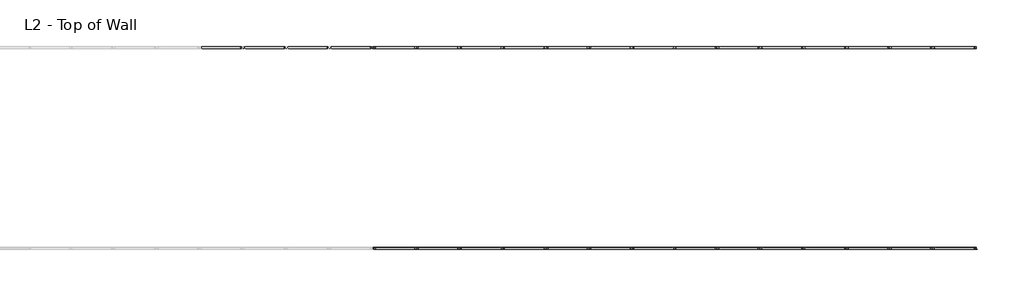
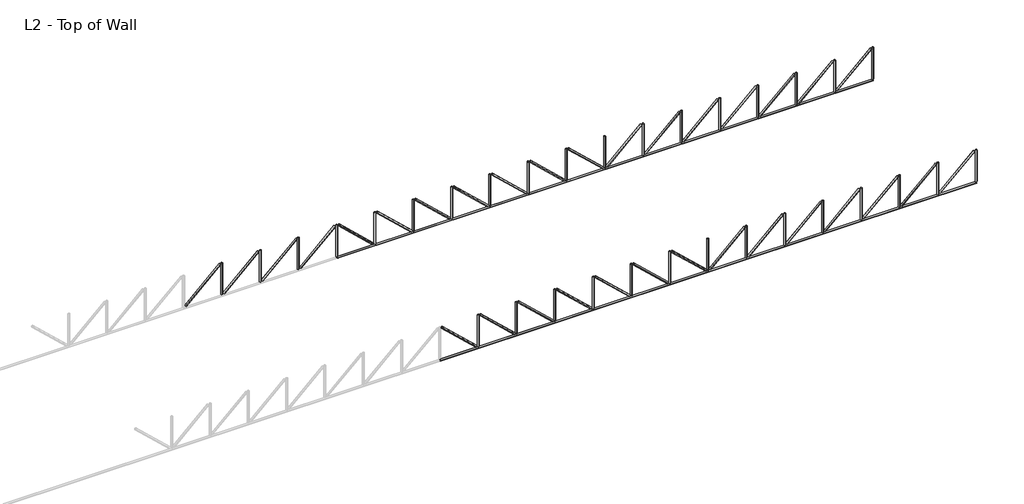
# One storey, part 4 of 4: 98 beams.
"""IFC4 building model written with IfcOpenShell, lengths in millimetres."""

import ifcopenshell
import ifcopenshell.guid

model = None  # the IFC model being written
_history = None  # IfcOwnerHistory: only IFC2X3 demands one
_inside = {}  # id of a spatial element -> (the spatial element, [elements in it])
_under = {}  # id of a project, library or spatial element -> (it, [spatial elements below it])
_declared = {}  # id of a project -> (the project, [libraries it declares])
_typed = {}  # id of a type object -> (the type object, [elements of that type])
_made_of = {}  # id of a material, layer set ... -> (it, [elements and type objects made of it])


def new_model(schema):
    """Start an empty IFC model of exactly this schema.

    Asked for "IFC4X3", IfcOpenShell would pick the latest addendum, in which some entities
    have other attributes; the version numbers below select the first issue.
    IFC2X3 requires an IfcOwnerHistory on every rooted entity: one is made here for all.
    """
    global model, _history
    if schema == "IFC4X3":
        model = ifcopenshell.file(schema_version=(4, 3, 0, 0))
    else:
        model = ifcopenshell.file(schema=schema)
    _inside.clear()
    _under.clear()
    _declared.clear()
    _typed.clear()
    _made_of.clear()
    _history = None
    if model.schema == "IFC2X3":
        org = make("IfcOrganization", Name="unknown")
        user = make(
            "IfcPersonAndOrganization",
            ThePerson=make("IfcPerson", FamilyName="unknown"),
            TheOrganization=org,
        )
        app = make(
            "IfcApplication",
            ApplicationDeveloper=org,
            Version="unknown",
            ApplicationFullName="unknown",
            ApplicationIdentifier="unknown",
        )
        _history = make(
            "IfcOwnerHistory",
            OwningUser=user,
            OwningApplication=app,
            ChangeAction="ADDED",
            CreationDate=0,
        )
    return model


def make(cls, **values):
    """One entity of the class cls with the attributes given. An attribute that is None is left unset."""
    return model.create_entity(
        cls, **{name: value for name, value in values.items() if value is not None}
    )


def rooted(cls, **values):
    """An entity with a GlobalId (a new one), such as an element, a storey or a relation."""
    return make(cls, GlobalId=ifcopenshell.guid.new(), OwnerHistory=_history, **values)


def si_unit(unit_type, name, prefix=None):
    """IfcSIUnit, for example si_unit("LENGTHUNIT", "METRE", prefix="MILLI")."""
    return make("IfcSIUnit", UnitType=unit_type, Prefix=prefix, Name=name)


def assignment(units):
    """IfcUnitAssignment: the units of a project."""
    return None if units is None else make("IfcUnitAssignment", Units=units)


def point(xyz):
    """IfcCartesianPoint."""
    return None if xyz is None else make("IfcCartesianPoint", Coordinates=xyz)


def direction(xyz):
    """IfcDirection."""
    return None if xyz is None else make("IfcDirection", DirectionRatios=xyz)


def frame(location, z_axis=None, x_axis=None):
    """IfcAxis2Placement3D, a coordinate frame: its origin and axes. An axis left out is left unset."""
    return make(
        "IfcAxis2Placement3D",
        Location=point(location),
        Axis=direction(z_axis),
        RefDirection=direction(x_axis),
    )


def frame_2d(location, x_axis=None):
    """IfcAxis2Placement2D, a coordinate frame in the plane: its origin and x axis."""
    return make(
        "IfcAxis2Placement2D", Location=point(location), RefDirection=direction(x_axis)
    )


def origin():
    """The frame at (0, 0, 0) with its axes left unset."""
    return frame((0.0, 0.0, 0.0))


def origin_2d():
    """The frame at (0, 0) in the plane with its x axis left unset."""
    return frame_2d((0.0, 0.0))


def place(relative_to, where):
    """IfcLocalPlacement: puts the frame where relative to a parent placement (None: the world)."""
    return make(
        "IfcLocalPlacement", PlacementRelTo=relative_to, RelativePlacement=where
    )


def context(
    kind, dimensions, precision=None, world=None, true_north=None, identifier=None
):
    """IfcGeometricRepresentationContext, for example the 3D "Model" context."""
    return make(
        "IfcGeometricRepresentationContext",
        ContextIdentifier=identifier,
        ContextType=kind,
        CoordinateSpaceDimension=dimensions,
        Precision=precision,
        WorldCoordinateSystem=world,
        TrueNorth=true_north,
    )


def project(units=None, contexts=None):
    """IfcProject with its units and contexts."""
    return rooted(
        "IfcProject",
        Name="project",
        RepresentationContexts=contexts,
        UnitsInContext=assignment(units),
    )


def spatial(cls, under=None, at=None, **own):
    """A site, building, storey or space (cls), placed at a placement, below another one or the project."""
    s = rooted(cls, ObjectPlacement=at, **own)
    if under is not None:
        _under.setdefault(under.id(), (under, []))[1].append(s)
    return s


def circle_curve(where, radius):
    """IfcCircle in the frame where."""
    return make("IfcCircle", Position=where, Radius=radius)


def trimmed(basis, trim1, trim2, sense, master):
    """IfcTrimmedCurve: the piece of a basis curve between two trims."""
    return make(
        "IfcTrimmedCurve",
        BasisCurve=basis,
        Trim1=trim1,
        Trim2=trim2,
        SenseAgreement=sense,
        MasterRepresentation=master,
    )


def segment(curve, same_sense, transition):
    """IfcCompositeCurveSegment."""
    return make(
        "IfcCompositeCurveSegment",
        Transition=transition,
        SameSense=same_sense,
        ParentCurve=curve,
    )


def composite_curve(segments, self_intersect=None):
    """IfcCompositeCurve: segments joined end to end."""
    return make("IfcCompositeCurve", Segments=segments, SelfIntersect=self_intersect)


def outline(outer, holes=None, kind="AREA"):
    """IfcArbitraryClosedProfileDef: a profile drawn as a closed curve; with holes, ...WithVoids."""
    if holes is None:
        return make("IfcArbitraryClosedProfileDef", ProfileType=kind, OuterCurve=outer)
    return make(
        "IfcArbitraryProfileDefWithVoids",
        ProfileType=kind,
        OuterCurve=outer,
        InnerCurves=holes,
    )


def extrude(swept, where, along, depth):
    """IfcExtrudedAreaSolid: the profile swept, set in the frame where, extruded along a direction by depth."""
    return make(
        "IfcExtrudedAreaSolid",
        SweptArea=swept,
        Position=where,
        ExtrudedDirection=direction(along),
        Depth=depth,
    )


def shape(context_of_items, identifier, shape_type, items):
    """IfcShapeRepresentation: the items that make up one representation, for example the "Body"."""
    return make(
        "IfcShapeRepresentation",
        ContextOfItems=context_of_items,
        RepresentationIdentifier=identifier,
        RepresentationType=shape_type,
        Items=items,
    )


def source(mapping_origin, context_of_items, identifier, shape_type, items):
    """IfcRepresentationMap: a shape defined once, which mapped items show again and again."""
    return make(
        "IfcRepresentationMap",
        MappingOrigin=mapping_origin,
        MappedRepresentation=shape(context_of_items, identifier, shape_type, items),
    )


def transform(
    local_origin,
    x_axis=None,
    y_axis=None,
    z_axis=None,
    scale=None,
    scale2=None,
    scale3=None,
    uniform=True,
):
    """IfcCartesianTransformationOperator3D, or its non-uniform kind. x_axis, y_axis, z_axis: its Axis1, 2, 3."""
    if uniform:
        return make(
            "IfcCartesianTransformationOperator3D",
            Axis1=direction(x_axis),
            Axis2=direction(y_axis),
            LocalOrigin=point(local_origin),
            Scale=scale,
            Axis3=direction(z_axis),
        )
    return make(
        "IfcCartesianTransformationOperator3DnonUniform",
        Axis1=direction(x_axis),
        Axis2=direction(y_axis),
        LocalOrigin=point(local_origin),
        Scale=scale,
        Axis3=direction(z_axis),
        Scale2=scale2,
        Scale3=scale3,
    )


def mapped(mapping_source, mapping_target):
    """IfcMappedItem: shows the shape of a source again, moved by a transform."""
    return make(
        "IfcMappedItem", MappingSource=mapping_source, MappingTarget=mapping_target
    )


def made_of(thing, what):
    """Note that an element or type object is made of a material, layer set ...; save() writes the relation."""
    if what is not None:
        _made_of.setdefault(what.id(), (what, []))[1].append(thing)
    return thing


def element(
    cls,
    number,
    at=None,
    inside=None,
    cuts=None,
    type_object=None,
    material=None,
    context=None,
    identifier="Body",
    shape_type=None,
    held_by="IfcProductDefinitionShape",
    body=None,
    shapes=None,
    **own,
):
    """One element of the class cls, such as IfcWall. Its Tag is "e" and its number.

    at: its placement. inside: the storey or other place that contains it. cuts: it is an
    opening in that element (IfcRelVoidsElement). A single representation is given by context,
    identifier, shape_type and body (its items); several are given by shapes. held_by: the class
    of the entity that holds the representations. save() writes the other relations.
    """
    e = rooted(cls, Tag="e%d" % number, ObjectPlacement=at, **own)
    if body is not None:
        shapes = [shape(context, identifier, shape_type, body)]
    if shapes is not None:
        e.Representation = make(held_by, Representations=shapes)
    if inside is not None:
        _inside.setdefault(inside.id(), (inside, []))[1].append(e)
    if cuts is not None:
        rooted(
            "IfcRelVoidsElement", RelatingBuildingElement=cuts, RelatedOpeningElement=e
        )
    if type_object is not None:
        _typed.setdefault(type_object.id(), (type_object, []))[1].append(e)
    return made_of(e, material)


def aggregate(whole, parts):
    """IfcRelAggregates: a whole, such as a stair, and the parts it consists of."""
    return rooted("IfcRelAggregates", RelatingObject=whole, RelatedObjects=parts)


def save(model, path):
    """Write the relations noted so far, then the file.

    IfcRelAggregates (storeys below a building ...), IfcRelContainedInSpatialStructure (elements
    in a storey), IfcRelDefinesByType, IfcRelAssociatesMaterial and IfcRelDeclares: one each for
    every whole, place, type object, material and project.
    """
    for whole, parts in _under.values():
        aggregate(whole, parts)
    for where, things in _inside.values():
        rooted(
            "IfcRelContainedInSpatialStructure",
            RelatedElements=things,
            RelatingStructure=where,
        )
    for kind, things in _typed.values():
        rooted("IfcRelDefinesByType", RelatedObjects=things, RelatingType=kind)
    for what, things in _made_of.values():
        rooted("IfcRelAssociatesMaterial", RelatedObjects=things, RelatingMaterial=what)
    for by, libraries in _declared.values():
        rooted("IfcRelDeclares", RelatingContext=by, RelatedDefinitions=libraries)
    model.write(path)


def circular_hollow_sections_chs60_3x5_c94bd862(model_context):
    return source(origin(), model_context, "Body", "SweptSolid", [
        extrude(outline(composite_curve([segment(trimmed(circle_curve(origin_2d(), 30.15), [point((-30.15, 0.0))], [point((30.15, 0.0))], False, "CARTESIAN"), True, "CONTINUOUS"), segment(trimmed(circle_curve(origin_2d(), 30.15), [point((30.15, 0.0))], [point((-30.15, 0.0))], False, "CARTESIAN"), True, "CONTINUOUS")], self_intersect=False), holes=[composite_curve([segment(trimmed(circle_curve(origin_2d(), 25.15), [point((25.15, 0.0))], [point((-25.15, 0.0))], True, "CARTESIAN"), True, "CONTINUOUS"), segment(trimmed(circle_curve(origin_2d(), 25.15), [point((-25.15, 0.0))], [point((25.15, 0.0))], True, "CARTESIAN"), True, "CONTINUOUS")], self_intersect=False)]), frame((-557.0, 0.0, 0.0), z_axis=(1.0, 0.0, 0.0), x_axis=(0.0, 1.0, 0.0)), (0.0, 0.0, 1.0), 1114.0),
    ])


def circular_hollow_sections_chs60_3x5_b8a643cb(model_context):
    return source(origin(), model_context, "Body", "SweptSolid", [
        extrude(outline(composite_curve([segment(trimmed(circle_curve(origin_2d(), 30.15), [point((-30.15, 0.0))], [point((30.15, 0.0))], False, "CARTESIAN"), True, "CONTINUOUS"), segment(trimmed(circle_curve(origin_2d(), 30.15), [point((30.15, 0.0))], [point((-30.15, 0.0))], False, "CARTESIAN"), True, "CONTINUOUS")], self_intersect=False), holes=[composite_curve([segment(trimmed(circle_curve(origin_2d(), 25.15), [point((25.15, 0.0))], [point((-25.15, 0.0))], True, "CARTESIAN"), True, "CONTINUOUS"), segment(trimmed(circle_curve(origin_2d(), 25.15), [point((-25.15, 0.0))], [point((25.15, 0.0))], True, "CARTESIAN"), True, "CONTINUOUS")], self_intersect=False)]), frame((-790.0, 0.0, 0.0), z_axis=(1.0, 0.0, 0.0), x_axis=(0.0, 1.0, 0.0)), (0.0, 0.0, 1.0), 1580.0),
    ])


def circular_hollow_sections_chs60_3x5_ee2473de(model_context):
    return source(origin(), model_context, "Body", "SweptSolid", [
        extrude(outline(composite_curve([segment(trimmed(circle_curve(origin_2d(), 30.15), [point((-30.15, 0.0))], [point((30.15, 0.0))], False, "CARTESIAN"), True, "CONTINUOUS"), segment(trimmed(circle_curve(origin_2d(), 30.15), [point((30.15, 0.0))], [point((-30.15, 0.0))], False, "CARTESIAN"), True, "CONTINUOUS")], self_intersect=False), holes=[composite_curve([segment(trimmed(circle_curve(origin_2d(), 25.15), [point((25.15, 0.0))], [point((-25.15, 0.0))], True, "CARTESIAN"), True, "CONTINUOUS"), segment(trimmed(circle_curve(origin_2d(), 25.15), [point((-25.15, 0.0))], [point((25.15, 0.0))], True, "CARTESIAN"), True, "CONTINUOUS")], self_intersect=False)]), frame((-9000.0, 0.0, 0.0), z_axis=(1.0, 0.0, 0.0), x_axis=(0.0, 1.0, 0.0)), (0.0, 0.0, 1.0), 18000.0),
    ])


def circular_hollow_sections_chs60_3x5_7809bf4e(model_context):
    return source(origin(), model_context, "Body", "SweptSolid", [
        extrude(outline(composite_curve([segment(trimmed(circle_curve(origin_2d(), 30.15), [point((-30.15, 0.0))], [point((30.15, 0.0))], False, "CARTESIAN"), True, "CONTINUOUS"), segment(trimmed(circle_curve(origin_2d(), 30.15), [point((30.15, 0.0))], [point((-30.15, 0.0))], False, "CARTESIAN"), True, "CONTINUOUS")], self_intersect=False), holes=[composite_curve([segment(trimmed(circle_curve(origin_2d(), 25.15), [point((25.15, 0.0))], [point((-25.15, 0.0))], True, "CARTESIAN"), True, "CONTINUOUS"), segment(trimmed(circle_curve(origin_2d(), 25.15), [point((-25.15, 0.0))], [point((25.15, 0.0))], True, "CARTESIAN"), True, "CONTINUOUS")], self_intersect=False)]), frame((-600.0, 0.0, 0.0), z_axis=(1.0, 0.0, 0.0), x_axis=(0.0, 1.0, 0.0)), (0.0, 0.0, 1.0), 1157.0),
    ])


model = new_model("IFC4")

# Units and contexts
model_context = context("Model", 3, world=origin())
ifc_project = project(units=[si_unit("LENGTHUNIT", "METRE", prefix="MILLI")], contexts=[model_context])

# Site, building, storey
site = spatial("IfcSite", under=ifc_project)
building = spatial("IfcBuilding", under=site)
storey = spatial("IfcBuildingStorey", under=building, Name="L2 - Top of Wall", Elevation=6600.0)

# Beams
placement = place(None, origin())
circular_hollow_sections_chs60_3x5_shape = circular_hollow_sections_chs60_3x5_c94bd862(model_context)
element("IfcBeam", 1, ObjectType="Circular Hollow Sections : CHS60.3x5", at=placement, inside=storey, context=model_context, shape_type="MappedRepresentation", body=[
    mapped(circular_hollow_sections_chs60_3x5_shape, transform((27576.1803686, 6941.2380918, 7200.0), x_axis=(0.0, 0.0, 1.0), y_axis=(0.0, -1.0, 0.0), z_axis=(1.0, 0.0, 0.0))),
])
element("IfcBeam", 2, ObjectType="Circular Hollow Sections : CHS60.3x5", at=placement, inside=storey, context=model_context, shape_type="MappedRepresentation", body=[
    mapped(circular_hollow_sections_chs60_3x5_shape, transform((26290.4660829, 6941.2380918, 7200.0), x_axis=(0.0, 0.0, 1.0), y_axis=(0.0, -1.0, 0.0), z_axis=(1.0, 0.0, 0.0))),
])
element("IfcBeam", 3, ObjectType="Circular Hollow Sections : CHS60.3x5", at=placement, inside=storey, context=model_context, shape_type="MappedRepresentation", body=[
    mapped(circular_hollow_sections_chs60_3x5_shape, transform((25004.7517972, 6941.2380918, 7200.0), x_axis=(0.0, 0.0, 1.0), y_axis=(0.0, -1.0, 0.0), z_axis=(1.0, 0.0, 0.0))),
])
element("IfcBeam", 4, ObjectType="Circular Hollow Sections : CHS60.3x5", at=placement, inside=storey, context=model_context, shape_type="MappedRepresentation", body=[
    mapped(circular_hollow_sections_chs60_3x5_shape, transform((28861.8946543, 6941.2380918, 7200.0), x_axis=(0.0, 0.0, 1.0), y_axis=(0.0, -1.0, 0.0), z_axis=(1.0, 0.0, 0.0))),
])
element("IfcBeam", 5, ObjectType="Circular Hollow Sections : CHS60.3x5", at=placement, inside=storey, context=model_context, shape_type="MappedRepresentation", body=[
    mapped(circular_hollow_sections_chs60_3x5_shape, transform((45576.1803686, 6941.2380918, 7200.0), x_axis=(0.0, 0.0, 1.0), y_axis=(0.0, -1.0, 0.0), z_axis=(1.0, 0.0, 0.0))),
])
element("IfcBeam", 6, ObjectType="Circular Hollow Sections : CHS60.3x5", at=placement, inside=storey, context=model_context, shape_type="MappedRepresentation", body=[
    mapped(circular_hollow_sections_chs60_3x5_shape, transform((30147.60894, 6941.2380918, 7200.0), x_axis=(0.0, 0.0, 1.0), y_axis=(0.0, -1.0, 0.0), z_axis=(1.0, 0.0, 0.0))),
])
element("IfcBeam", 7, ObjectType="Circular Hollow Sections : CHS60.3x5", at=placement, inside=storey, context=model_context, shape_type="MappedRepresentation", body=[
    mapped(circular_hollow_sections_chs60_3x5_shape, transform((44290.4660829, 6941.2380918, 7200.0), x_axis=(0.0, 0.0, 1.0), y_axis=(0.0, -1.0, 0.0), z_axis=(1.0, 0.0, 0.0))),
])
element("IfcBeam", 8, ObjectType="Circular Hollow Sections : CHS60.3x5", at=placement, inside=storey, context=model_context, shape_type="MappedRepresentation", body=[
    mapped(circular_hollow_sections_chs60_3x5_shape, transform((31433.3232257, 6941.2380918, 7200.0), x_axis=(0.0, 0.0, 1.0), y_axis=(0.0, -1.0, 0.0), z_axis=(1.0, 0.0, 0.0))),
])
element("IfcBeam", 9, ObjectType="Circular Hollow Sections : CHS60.3x5", at=placement, inside=storey, context=model_context, shape_type="MappedRepresentation", body=[
    mapped(circular_hollow_sections_chs60_3x5_shape, transform((43004.7517972, 6941.2380918, 7200.0), x_axis=(0.0, 0.0, 1.0), y_axis=(0.0, -1.0, 0.0), z_axis=(1.0, 0.0, 0.0))),
])
element("IfcBeam", 10, ObjectType="Circular Hollow Sections : CHS60.3x5", at=placement, inside=storey, context=model_context, shape_type="MappedRepresentation", body=[
    mapped(circular_hollow_sections_chs60_3x5_shape, transform((32719.0375115, 6941.2380918, 7200.0), x_axis=(0.0, 0.0, 1.0), y_axis=(0.0, -1.0, 0.0), z_axis=(1.0, 0.0, 0.0))),
])
element("IfcBeam", 11, ObjectType="Circular Hollow Sections : CHS60.3x5", at=placement, inside=storey, context=model_context, shape_type="MappedRepresentation", body=[
    mapped(circular_hollow_sections_chs60_3x5_shape, transform((41719.0375115, 6941.2380918, 7200.0), x_axis=(0.0, 0.0, 1.0), y_axis=(0.0, -1.0, 0.0), z_axis=(1.0, 0.0, 0.0))),
])
element("IfcBeam", 12, ObjectType="Circular Hollow Sections : CHS60.3x5", at=placement, inside=storey, context=model_context, shape_type="MappedRepresentation", body=[
    mapped(circular_hollow_sections_chs60_3x5_shape, transform((40433.3232257, 6941.2380918, 7200.0), x_axis=(0.0, 0.0, 1.0), y_axis=(0.0, -1.0, 0.0), z_axis=(1.0, 0.0, 0.0))),
])
element("IfcBeam", 13, ObjectType="Circular Hollow Sections : CHS60.3x5", at=placement, inside=storey, context=model_context, shape_type="MappedRepresentation", body=[
    mapped(circular_hollow_sections_chs60_3x5_shape, transform((46861.8946543, 6941.2380918, 7200.0), x_axis=(0.0, 0.0, 1.0), y_axis=(0.0, -1.0, 0.0), z_axis=(1.0, 0.0, 0.0))),
])
element("IfcBeam", 14, ObjectType="Circular Hollow Sections : CHS60.3x5", at=placement, inside=storey, context=model_context, shape_type="MappedRepresentation", body=[
    mapped(circular_hollow_sections_chs60_3x5_shape, transform((39147.60894, 6941.2380918, 7200.0), x_axis=(0.0, 0.0, 1.0), y_axis=(0.0, -1.0, 0.0), z_axis=(1.0, 0.0, 0.0))),
])
element("IfcBeam", 15, ObjectType="Circular Hollow Sections : CHS60.3x5", at=placement, inside=storey, context=model_context, shape_type="MappedRepresentation", body=[
    mapped(circular_hollow_sections_chs60_3x5_shape, transform((34004.7517972, 6941.2380918, 7200.0), x_axis=(0.0, 0.0, 1.0), y_axis=(0.0, -1.0, 0.0), z_axis=(1.0, 0.0, 0.0))),
])
element("IfcBeam", 16, ObjectType="Circular Hollow Sections : CHS60.3x5", at=placement, inside=storey, context=model_context, shape_type="MappedRepresentation", body=[
    mapped(circular_hollow_sections_chs60_3x5_shape, transform((35290.4660829, 6941.2380918, 7200.0), x_axis=(0.0, 0.0, 1.0), y_axis=(0.0, -1.0, 0.0), z_axis=(1.0, 0.0, 0.0))),
])
element("IfcBeam", 17, ObjectType="Circular Hollow Sections : CHS60.3x5", at=placement, inside=storey, context=model_context, shape_type="MappedRepresentation", body=[
    mapped(circular_hollow_sections_chs60_3x5_shape, transform((36576.1803686, 6941.2380918, 7200.0), x_axis=(0.0, 0.0, 1.0), y_axis=(0.0, -1.0, 0.0), z_axis=(1.0, 0.0, 0.0))),
])
element("IfcBeam", 18, ObjectType="Circular Hollow Sections : CHS60.3x5", at=placement, inside=storey, context=model_context, shape_type="MappedRepresentation", body=[
    mapped(circular_hollow_sections_chs60_3x5_shape, transform((37861.8946543, 6941.2380918, 7200.0), x_axis=(0.0, 0.0, 1.0), y_axis=(0.0, -1.0, 0.0), z_axis=(1.0, 0.0, 0.0))),
])
element("IfcBeam", 19, ObjectType="Circular Hollow Sections : CHS60.3x5", at=placement, inside=storey, context=model_context, shape_type="MappedRepresentation", body=[
    mapped(circular_hollow_sections_chs60_3x5_shape, transform((45576.1803686, 6941.2380918, 7200.0), x_axis=(0.0, 0.0, 1.0), y_axis=(0.0, -1.0, 0.0), z_axis=(1.0, 0.0, 0.0))),
])
element("IfcBeam", 20, ObjectType="Circular Hollow Sections : CHS60.3x5", at=placement, inside=storey, context=model_context, shape_type="MappedRepresentation", body=[
    mapped(circular_hollow_sections_chs60_3x5_shape, transform((30147.60894, 6941.2380918, 7200.0), x_axis=(0.0, 0.0, 1.0), y_axis=(0.0, -1.0, 0.0), z_axis=(1.0, 0.0, 0.0))),
])
element("IfcBeam", 21, ObjectType="Circular Hollow Sections : CHS60.3x5", at=placement, inside=storey, context=model_context, shape_type="MappedRepresentation", body=[
    mapped(circular_hollow_sections_chs60_3x5_shape, transform((44290.4660829, 6941.2380918, 7200.0), x_axis=(0.0, 0.0, 1.0), y_axis=(0.0, -1.0, 0.0), z_axis=(1.0, 0.0, 0.0))),
])
element("IfcBeam", 22, ObjectType="Circular Hollow Sections : CHS60.3x5", at=placement, inside=storey, context=model_context, shape_type="MappedRepresentation", body=[
    mapped(circular_hollow_sections_chs60_3x5_shape, transform((31433.3232257, 6941.2380918, 7200.0), x_axis=(0.0, 0.0, 1.0), y_axis=(0.0, -1.0, 0.0), z_axis=(1.0, 0.0, 0.0))),
])
element("IfcBeam", 23, ObjectType="Circular Hollow Sections : CHS60.3x5", at=placement, inside=storey, context=model_context, shape_type="MappedRepresentation", body=[
    mapped(circular_hollow_sections_chs60_3x5_shape, transform((43004.7517972, 6941.2380918, 7200.0), x_axis=(0.0, 0.0, 1.0), y_axis=(0.0, -1.0, 0.0), z_axis=(1.0, 0.0, 0.0))),
])
element("IfcBeam", 24, ObjectType="Circular Hollow Sections : CHS60.3x5", at=placement, inside=storey, context=model_context, shape_type="MappedRepresentation", body=[
    mapped(circular_hollow_sections_chs60_3x5_shape, transform((32719.0375115, 6941.2380918, 7200.0), x_axis=(0.0, 0.0, 1.0), y_axis=(0.0, -1.0, 0.0), z_axis=(1.0, 0.0, 0.0))),
])
element("IfcBeam", 25, ObjectType="Circular Hollow Sections : CHS60.3x5", at=placement, inside=storey, context=model_context, shape_type="MappedRepresentation", body=[
    mapped(circular_hollow_sections_chs60_3x5_shape, transform((41719.0375115, 6941.2380918, 7200.0), x_axis=(0.0, 0.0, 1.0), y_axis=(0.0, -1.0, 0.0), z_axis=(1.0, 0.0, 0.0))),
])
element("IfcBeam", 26, ObjectType="Circular Hollow Sections : CHS60.3x5", at=placement, inside=storey, context=model_context, shape_type="MappedRepresentation", body=[
    mapped(circular_hollow_sections_chs60_3x5_shape, transform((40433.3232257, 6941.2380918, 7200.0), x_axis=(0.0, 0.0, 1.0), y_axis=(0.0, -1.0, 0.0), z_axis=(1.0, 0.0, 0.0))),
])
element("IfcBeam", 27, ObjectType="Circular Hollow Sections : CHS60.3x5", at=placement, inside=storey, context=model_context, shape_type="MappedRepresentation", body=[
    mapped(circular_hollow_sections_chs60_3x5_shape, transform((46861.8946543, 6941.2380918, 7200.0), x_axis=(0.0, 0.0, 1.0), y_axis=(0.0, -1.0, 0.0), z_axis=(1.0, 0.0, 0.0))),
])
element("IfcBeam", 28, ObjectType="Circular Hollow Sections : CHS60.3x5", at=placement, inside=storey, context=model_context, shape_type="MappedRepresentation", body=[
    mapped(circular_hollow_sections_chs60_3x5_shape, transform((39147.60894, 6941.2380918, 7200.0), x_axis=(0.0, 0.0, 1.0), y_axis=(0.0, -1.0, 0.0), z_axis=(1.0, 0.0, 0.0))),
])
element("IfcBeam", 29, ObjectType="Circular Hollow Sections : CHS60.3x5", at=placement, inside=storey, context=model_context, shape_type="MappedRepresentation", body=[
    mapped(circular_hollow_sections_chs60_3x5_shape, transform((34004.7517972, 6941.2380918, 7200.0), x_axis=(0.0, 0.0, 1.0), y_axis=(0.0, -1.0, 0.0), z_axis=(1.0, 0.0, 0.0))),
])
element("IfcBeam", 30, ObjectType="Circular Hollow Sections : CHS60.3x5", at=placement, inside=storey, context=model_context, shape_type="MappedRepresentation", body=[
    mapped(circular_hollow_sections_chs60_3x5_shape, transform((35290.4660829, 6941.2380918, 7200.0), x_axis=(0.0, 0.0, 1.0), y_axis=(0.0, -1.0, 0.0), z_axis=(1.0, 0.0, 0.0))),
])
element("IfcBeam", 31, ObjectType="Circular Hollow Sections : CHS60.3x5", at=placement, inside=storey, context=model_context, shape_type="MappedRepresentation", body=[
    mapped(circular_hollow_sections_chs60_3x5_shape, transform((36576.1803686, 6941.2380918, 7200.0), x_axis=(0.0, 0.0, 1.0), y_axis=(0.0, -1.0, 0.0), z_axis=(1.0, 0.0, 0.0))),
])
element("IfcBeam", 32, ObjectType="Circular Hollow Sections : CHS60.3x5", at=placement, inside=storey, context=model_context, shape_type="MappedRepresentation", body=[
    mapped(circular_hollow_sections_chs60_3x5_shape, transform((37861.8946543, 6941.2380918, 7200.0), x_axis=(0.0, 0.0, 1.0), y_axis=(0.0, -1.0, 0.0), z_axis=(1.0, 0.0, 0.0))),
])
element("IfcBeam", 33, ObjectType="Circular Hollow Sections : CHS60.3x5", at=placement, inside=storey, context=model_context, shape_type="MappedRepresentation", body=[
    mapped(circular_hollow_sections_chs60_3x5_shape, transform((45576.1803686, 941.2380918, 7200.0), x_axis=(0.0, 0.0, 1.0000000000000002), y_axis=(0.0, -1.0000000000000002, 0.0), z_axis=(1.0000000000000002, 0.0, 0.0))),
])
element("IfcBeam", 34, ObjectType="Circular Hollow Sections : CHS60.3x5", at=placement, inside=storey, context=model_context, shape_type="MappedRepresentation", body=[
    mapped(circular_hollow_sections_chs60_3x5_shape, transform((30147.60894, 941.2380918, 7200.0), x_axis=(0.0, 0.0, 1.0000000000000002), y_axis=(0.0, -1.0000000000000002, 0.0), z_axis=(1.0000000000000002, 0.0, 0.0))),
])
element("IfcBeam", 35, ObjectType="Circular Hollow Sections : CHS60.3x5", at=placement, inside=storey, context=model_context, shape_type="MappedRepresentation", body=[
    mapped(circular_hollow_sections_chs60_3x5_shape, transform((44290.4660829, 941.2380918, 7200.0), x_axis=(0.0, 0.0, 1.0000000000000002), y_axis=(0.0, -1.0000000000000002, 0.0), z_axis=(1.0000000000000002, 0.0, 0.0))),
])
element("IfcBeam", 36, ObjectType="Circular Hollow Sections : CHS60.3x5", at=placement, inside=storey, context=model_context, shape_type="MappedRepresentation", body=[
    mapped(circular_hollow_sections_chs60_3x5_shape, transform((31433.3232257, 941.2380918, 7200.0), x_axis=(0.0, 0.0, 1.0000000000000002), y_axis=(0.0, -1.0000000000000002, 0.0), z_axis=(1.0000000000000002, 0.0, 0.0))),
])
element("IfcBeam", 37, ObjectType="Circular Hollow Sections : CHS60.3x5", at=placement, inside=storey, context=model_context, shape_type="MappedRepresentation", body=[
    mapped(circular_hollow_sections_chs60_3x5_shape, transform((43004.7517972, 941.2380918, 7200.0), x_axis=(0.0, 0.0, 1.0000000000000002), y_axis=(0.0, -1.0000000000000002, 0.0), z_axis=(1.0000000000000002, 0.0, 0.0))),
])
element("IfcBeam", 38, ObjectType="Circular Hollow Sections : CHS60.3x5", at=placement, inside=storey, context=model_context, shape_type="MappedRepresentation", body=[
    mapped(circular_hollow_sections_chs60_3x5_shape, transform((32719.0375115, 941.2380918, 7200.0), x_axis=(0.0, 0.0, 1.0000000000000002), y_axis=(0.0, -1.0000000000000002, 0.0), z_axis=(1.0000000000000002, 0.0, 0.0))),
])
element("IfcBeam", 39, ObjectType="Circular Hollow Sections : CHS60.3x5", at=placement, inside=storey, context=model_context, shape_type="MappedRepresentation", body=[
    mapped(circular_hollow_sections_chs60_3x5_shape, transform((41719.0375115, 941.2380918, 7200.0), x_axis=(0.0, 0.0, 1.0000000000000002), y_axis=(0.0, -1.0000000000000002, 0.0), z_axis=(1.0000000000000002, 0.0, 0.0))),
])
element("IfcBeam", 40, ObjectType="Circular Hollow Sections : CHS60.3x5", at=placement, inside=storey, context=model_context, shape_type="MappedRepresentation", body=[
    mapped(circular_hollow_sections_chs60_3x5_shape, transform((40433.3232257, 941.2380918, 7200.0), x_axis=(0.0, 0.0, 1.0000000000000002), y_axis=(0.0, -1.0000000000000002, 0.0), z_axis=(1.0000000000000002, 0.0, 0.0))),
])
element("IfcBeam", 41, ObjectType="Circular Hollow Sections : CHS60.3x5", at=placement, inside=storey, context=model_context, shape_type="MappedRepresentation", body=[
    mapped(circular_hollow_sections_chs60_3x5_shape, transform((46861.8946543, 941.2380918, 7200.0), x_axis=(0.0, 0.0, 1.0000000000000002), y_axis=(0.0, -1.0000000000000002, 0.0), z_axis=(1.0000000000000002, 0.0, 0.0))),
])
element("IfcBeam", 42, ObjectType="Circular Hollow Sections : CHS60.3x5", at=placement, inside=storey, context=model_context, shape_type="MappedRepresentation", body=[
    mapped(circular_hollow_sections_chs60_3x5_shape, transform((39147.60894, 941.2380918, 7200.0), x_axis=(0.0, 0.0, 1.0000000000000002), y_axis=(0.0, -1.0000000000000002, 0.0), z_axis=(1.0000000000000002, 0.0, 0.0))),
])
element("IfcBeam", 43, ObjectType="Circular Hollow Sections : CHS60.3x5", at=placement, inside=storey, context=model_context, shape_type="MappedRepresentation", body=[
    mapped(circular_hollow_sections_chs60_3x5_shape, transform((34004.7517972, 941.2380918, 7200.0), x_axis=(0.0, 0.0, 1.0000000000000002), y_axis=(0.0, -1.0000000000000002, 0.0), z_axis=(1.0000000000000002, 0.0, 0.0))),
])
element("IfcBeam", 44, ObjectType="Circular Hollow Sections : CHS60.3x5", at=placement, inside=storey, context=model_context, shape_type="MappedRepresentation", body=[
    mapped(circular_hollow_sections_chs60_3x5_shape, transform((35290.4660829, 941.2380918, 7200.0), x_axis=(0.0, 0.0, 1.0000000000000002), y_axis=(0.0, -1.0000000000000002, 0.0), z_axis=(1.0000000000000002, 0.0, 0.0))),
])
element("IfcBeam", 45, ObjectType="Circular Hollow Sections : CHS60.3x5", at=placement, inside=storey, context=model_context, shape_type="MappedRepresentation", body=[
    mapped(circular_hollow_sections_chs60_3x5_shape, transform((36576.1803686, 941.2380918, 7200.0), x_axis=(0.0, 0.0, 1.0000000000000002), y_axis=(0.0, -1.0000000000000002, 0.0), z_axis=(1.0000000000000002, 0.0, 0.0))),
])
element("IfcBeam", 46, ObjectType="Circular Hollow Sections : CHS60.3x5", at=placement, inside=storey, context=model_context, shape_type="MappedRepresentation", body=[
    mapped(circular_hollow_sections_chs60_3x5_shape, transform((37861.8946543, 941.2380918, 7200.0), x_axis=(0.0, 0.0, 1.0000000000000002), y_axis=(0.0, -1.0000000000000002, 0.0), z_axis=(1.0000000000000002, 0.0, 0.0))),
])
circular_hollow_sections_chs60_3x5_2_shape = circular_hollow_sections_chs60_3x5_b8a643cb(model_context)
element("IfcBeam", 47, ObjectType="Circular Hollow Sections : CHS60.3x5", at=placement, inside=storey, context=model_context, shape_type="MappedRepresentation", body=[
    mapped(circular_hollow_sections_chs60_3x5_2_shape, transform((26933.3232257, 6941.2380918, 7200.0), x_axis=(0.7310552682428697, 0.0, 0.6823182503600105), y_axis=(0.0, -1.0, 0.0), z_axis=(0.6823182503600105, 0.0, -0.7310552682428697))),
])
element("IfcBeam", 48, ObjectType="Circular Hollow Sections : CHS60.3x5", at=placement, inside=storey, context=model_context, shape_type="MappedRepresentation", body=[
    mapped(circular_hollow_sections_chs60_3x5_2_shape, transform((25647.60894, 6941.2380918, 7200.0), x_axis=(0.7310552682428697, 0.0, 0.6823182503600105), y_axis=(0.0, -1.0, 0.0), z_axis=(0.6823182503600105, 0.0, -0.7310552682428697))),
])
element("IfcBeam", 49, ObjectType="Circular Hollow Sections : CHS60.3x5", at=placement, inside=storey, context=model_context, shape_type="MappedRepresentation", body=[
    mapped(circular_hollow_sections_chs60_3x5_2_shape, transform((24361.8946543, 6941.2380918, 7200.0), x_axis=(0.7310552682428697, 0.0, 0.6823182503600105), y_axis=(0.0, -1.0, 0.0), z_axis=(0.6823182503600105, 0.0, -0.7310552682428697))),
])
element("IfcBeam", 50, ObjectType="Circular Hollow Sections : CHS60.3x5", at=placement, inside=storey, context=model_context, shape_type="MappedRepresentation", body=[
    mapped(circular_hollow_sections_chs60_3x5_2_shape, transform((28219.0375115, 6941.2380918, 7200.0), x_axis=(0.7310552682428697, 0.0, 0.6823182503600105), y_axis=(0.0, -1.0, 0.0), z_axis=(0.6823182503600105, 0.0, -0.7310552682428697))),
])
element("IfcBeam", 51, ObjectType="Circular Hollow Sections : CHS60.3x5", at=placement, inside=storey, context=model_context, shape_type="MappedRepresentation", body=[
    mapped(circular_hollow_sections_chs60_3x5_2_shape, transform((44933.3232257, 6941.2380918, 7200.0), x_axis=(0.7310552682428697, 0.0, 0.6823182503600105), y_axis=(0.0, -1.0, 0.0), z_axis=(0.6823182503600105, 0.0, -0.7310552682428697))),
])
element("IfcBeam", 52, ObjectType="Circular Hollow Sections : CHS60.3x5", at=placement, inside=storey, context=model_context, shape_type="MappedRepresentation", body=[
    mapped(circular_hollow_sections_chs60_3x5_2_shape, transform((30790.4660829, 6941.2380918, 7200.0), x_axis=(0.7310552682428686, 0.0, -0.6823182503600118), y_axis=(0.0, -1.0, 0.0), z_axis=(-0.6823182503600118, 0.0, -0.7310552682428686))),
])
element("IfcBeam", 53, ObjectType="Circular Hollow Sections : CHS60.3x5", at=placement, inside=storey, context=model_context, shape_type="MappedRepresentation", body=[
    mapped(circular_hollow_sections_chs60_3x5_2_shape, transform((43647.60894, 6941.2380918, 7200.0), x_axis=(0.7310552682428697, 0.0, 0.6823182503600105), y_axis=(0.0, -1.0, 0.0), z_axis=(0.6823182503600105, 0.0, -0.7310552682428697))),
])
element("IfcBeam", 54, ObjectType="Circular Hollow Sections : CHS60.3x5", at=placement, inside=storey, context=model_context, shape_type="MappedRepresentation", body=[
    mapped(circular_hollow_sections_chs60_3x5_2_shape, transform((32076.1803686, 6941.2380918, 7200.0), x_axis=(0.7310552682428686, 0.0, -0.6823182503600118), y_axis=(0.0, -1.0, 0.0), z_axis=(-0.6823182503600118, 0.0, -0.7310552682428686))),
])
element("IfcBeam", 55, ObjectType="Circular Hollow Sections : CHS60.3x5", at=placement, inside=storey, context=model_context, shape_type="MappedRepresentation", body=[
    mapped(circular_hollow_sections_chs60_3x5_2_shape, transform((42361.8946543, 6941.2380918, 7200.0), x_axis=(0.7310552682428697, 0.0, 0.6823182503600105), y_axis=(0.0, -1.0, 0.0), z_axis=(0.6823182503600105, 0.0, -0.7310552682428697))),
])
element("IfcBeam", 56, ObjectType="Circular Hollow Sections : CHS60.3x5", at=placement, inside=storey, context=model_context, shape_type="MappedRepresentation", body=[
    mapped(circular_hollow_sections_chs60_3x5_2_shape, transform((33361.8946543, 6941.2380918, 7200.0), x_axis=(0.7310552682428686, 0.0, -0.6823182503600118), y_axis=(0.0, -1.0, 0.0), z_axis=(-0.6823182503600118, 0.0, -0.7310552682428686))),
])
element("IfcBeam", 57, ObjectType="Circular Hollow Sections : CHS60.3x5", at=placement, inside=storey, context=model_context, shape_type="MappedRepresentation", body=[
    mapped(circular_hollow_sections_chs60_3x5_2_shape, transform((41076.1803686, 6941.2380918, 7200.0), x_axis=(0.7310552682428697, 0.0, 0.6823182503600105), y_axis=(0.0, -1.0, 0.0), z_axis=(0.6823182503600105, 0.0, -0.7310552682428697))),
])
element("IfcBeam", 58, ObjectType="Circular Hollow Sections : CHS60.3x5", at=placement, inside=storey, context=model_context, shape_type="MappedRepresentation", body=[
    mapped(circular_hollow_sections_chs60_3x5_2_shape, transform((39790.4660829, 6941.2380918, 7200.0), x_axis=(0.7310552682428697, 0.0, 0.6823182503600105), y_axis=(0.0, -1.0, 0.0), z_axis=(0.6823182503600105, 0.0, -0.7310552682428697))),
])
element("IfcBeam", 59, ObjectType="Circular Hollow Sections : CHS60.3x5", at=placement, inside=storey, context=model_context, shape_type="MappedRepresentation", body=[
    mapped(circular_hollow_sections_chs60_3x5_2_shape, transform((46219.0375115, 6941.2380918, 7200.0), x_axis=(0.7310552682428697, 0.0, 0.6823182503600105), y_axis=(0.0, -1.0, 0.0), z_axis=(0.6823182503600105, 0.0, -0.7310552682428697))),
])
element("IfcBeam", 60, ObjectType="Circular Hollow Sections : CHS60.3x5", at=placement, inside=storey, context=model_context, shape_type="MappedRepresentation", body=[
    mapped(circular_hollow_sections_chs60_3x5_2_shape, transform((38504.7517972, 6941.2380918, 7200.0), x_axis=(0.7310552682428697, 0.0, 0.6823182503600105), y_axis=(0.0, -1.0, 0.0), z_axis=(0.6823182503600105, 0.0, -0.7310552682428697))),
])
element("IfcBeam", 61, ObjectType="Circular Hollow Sections : CHS60.3x5", at=placement, inside=storey, context=model_context, shape_type="MappedRepresentation", body=[
    mapped(circular_hollow_sections_chs60_3x5_2_shape, transform((34647.60894, 6941.2380918, 7200.0), x_axis=(0.7310552682428686, 0.0, -0.6823182503600118), y_axis=(0.0, -1.0, 0.0), z_axis=(-0.6823182503600118, 0.0, -0.7310552682428686))),
])
element("IfcBeam", 62, ObjectType="Circular Hollow Sections : CHS60.3x5", at=placement, inside=storey, context=model_context, shape_type="MappedRepresentation", body=[
    mapped(circular_hollow_sections_chs60_3x5_2_shape, transform((35933.3232257, 6941.2380918, 7200.0), x_axis=(0.7310552682428686, 0.0, -0.6823182503600118), y_axis=(0.0, -1.0, 0.0), z_axis=(-0.6823182503600118, 0.0, -0.7310552682428686))),
])
element("IfcBeam", 63, ObjectType="Circular Hollow Sections : CHS60.3x5", at=placement, inside=storey, context=model_context, shape_type="MappedRepresentation", body=[
    mapped(circular_hollow_sections_chs60_3x5_2_shape, transform((29504.7517972, 6941.2380918, 7200.0), x_axis=(0.7310552682428686, 0.0, -0.6823182503600118), y_axis=(0.0, -1.0, 0.0), z_axis=(-0.6823182503600118, 0.0, -0.7310552682428686))),
])
element("IfcBeam", 64, ObjectType="Circular Hollow Sections : CHS60.3x5", at=placement, inside=storey, context=model_context, shape_type="MappedRepresentation", body=[
    mapped(circular_hollow_sections_chs60_3x5_2_shape, transform((37219.0375115, 6941.2380918, 7200.0), x_axis=(0.7310552682428686, 0.0, -0.6823182503600118), y_axis=(0.0, -1.0, 0.0), z_axis=(-0.6823182503600118, 0.0, -0.7310552682428686))),
])
element("IfcBeam", 65, ObjectType="Circular Hollow Sections : CHS60.3x5", at=placement, inside=storey, context=model_context, shape_type="MappedRepresentation", body=[
    mapped(circular_hollow_sections_chs60_3x5_2_shape, transform((44933.3232257, 6941.2380918, 7200.0), x_axis=(0.7310552682428697, 0.0, 0.6823182503600105), y_axis=(0.0, -1.0, 0.0), z_axis=(0.6823182503600105, 0.0, -0.7310552682428697))),
])
element("IfcBeam", 66, ObjectType="Circular Hollow Sections : CHS60.3x5", at=placement, inside=storey, context=model_context, shape_type="MappedRepresentation", body=[
    mapped(circular_hollow_sections_chs60_3x5_2_shape, transform((30790.4660829, 6941.2380918, 7200.0), x_axis=(0.7310552682428686, 0.0, -0.6823182503600118), y_axis=(0.0, -1.0, 0.0), z_axis=(-0.6823182503600118, 0.0, -0.7310552682428686))),
])
element("IfcBeam", 67, ObjectType="Circular Hollow Sections : CHS60.3x5", at=placement, inside=storey, context=model_context, shape_type="MappedRepresentation", body=[
    mapped(circular_hollow_sections_chs60_3x5_2_shape, transform((43647.60894, 6941.2380918, 7200.0), x_axis=(0.7310552682428697, 0.0, 0.6823182503600105), y_axis=(0.0, -1.0, 0.0), z_axis=(0.6823182503600105, 0.0, -0.7310552682428697))),
])
element("IfcBeam", 68, ObjectType="Circular Hollow Sections : CHS60.3x5", at=placement, inside=storey, context=model_context, shape_type="MappedRepresentation", body=[
    mapped(circular_hollow_sections_chs60_3x5_2_shape, transform((32076.1803686, 6941.2380918, 7200.0), x_axis=(0.7310552682428686, 0.0, -0.6823182503600118), y_axis=(0.0, -1.0, 0.0), z_axis=(-0.6823182503600118, 0.0, -0.7310552682428686))),
])
element("IfcBeam", 69, ObjectType="Circular Hollow Sections : CHS60.3x5", at=placement, inside=storey, context=model_context, shape_type="MappedRepresentation", body=[
    mapped(circular_hollow_sections_chs60_3x5_2_shape, transform((42361.8946543, 6941.2380918, 7200.0), x_axis=(0.7310552682428697, 0.0, 0.6823182503600105), y_axis=(0.0, -1.0, 0.0), z_axis=(0.6823182503600105, 0.0, -0.7310552682428697))),
])
element("IfcBeam", 70, ObjectType="Circular Hollow Sections : CHS60.3x5", at=placement, inside=storey, context=model_context, shape_type="MappedRepresentation", body=[
    mapped(circular_hollow_sections_chs60_3x5_2_shape, transform((33361.8946543, 6941.2380918, 7200.0), x_axis=(0.7310552682428686, 0.0, -0.6823182503600118), y_axis=(0.0, -1.0, 0.0), z_axis=(-0.6823182503600118, 0.0, -0.7310552682428686))),
])
element("IfcBeam", 71, ObjectType="Circular Hollow Sections : CHS60.3x5", at=placement, inside=storey, context=model_context, shape_type="MappedRepresentation", body=[
    mapped(circular_hollow_sections_chs60_3x5_2_shape, transform((41076.1803686, 6941.2380918, 7200.0), x_axis=(0.7310552682428697, 0.0, 0.6823182503600105), y_axis=(0.0, -1.0, 0.0), z_axis=(0.6823182503600105, 0.0, -0.7310552682428697))),
])
element("IfcBeam", 72, ObjectType="Circular Hollow Sections : CHS60.3x5", at=placement, inside=storey, context=model_context, shape_type="MappedRepresentation", body=[
    mapped(circular_hollow_sections_chs60_3x5_2_shape, transform((39790.4660829, 6941.2380918, 7200.0), x_axis=(0.7310552682428697, 0.0, 0.6823182503600105), y_axis=(0.0, -1.0, 0.0), z_axis=(0.6823182503600105, 0.0, -0.7310552682428697))),
])
element("IfcBeam", 73, ObjectType="Circular Hollow Sections : CHS60.3x5", at=placement, inside=storey, context=model_context, shape_type="MappedRepresentation", body=[
    mapped(circular_hollow_sections_chs60_3x5_2_shape, transform((46219.0375115, 6941.2380918, 7200.0), x_axis=(0.7310552682428697, 0.0, 0.6823182503600105), y_axis=(0.0, -1.0, 0.0), z_axis=(0.6823182503600105, 0.0, -0.7310552682428697))),
])
element("IfcBeam", 74, ObjectType="Circular Hollow Sections : CHS60.3x5", at=placement, inside=storey, context=model_context, shape_type="MappedRepresentation", body=[
    mapped(circular_hollow_sections_chs60_3x5_2_shape, transform((38504.7517972, 6941.2380918, 7200.0), x_axis=(0.7310552682428697, 0.0, 0.6823182503600105), y_axis=(0.0, -1.0, 0.0), z_axis=(0.6823182503600105, 0.0, -0.7310552682428697))),
])
element("IfcBeam", 75, ObjectType="Circular Hollow Sections : CHS60.3x5", at=placement, inside=storey, context=model_context, shape_type="MappedRepresentation", body=[
    mapped(circular_hollow_sections_chs60_3x5_2_shape, transform((34647.60894, 6941.2380918, 7200.0), x_axis=(0.7310552682428686, 0.0, -0.6823182503600118), y_axis=(0.0, -1.0, 0.0), z_axis=(-0.6823182503600118, 0.0, -0.7310552682428686))),
])
element("IfcBeam", 76, ObjectType="Circular Hollow Sections : CHS60.3x5", at=placement, inside=storey, context=model_context, shape_type="MappedRepresentation", body=[
    mapped(circular_hollow_sections_chs60_3x5_2_shape, transform((35933.3232257, 6941.2380918, 7200.0), x_axis=(0.7310552682428686, 0.0, -0.6823182503600118), y_axis=(0.0, -1.0, 0.0), z_axis=(-0.6823182503600118, 0.0, -0.7310552682428686))),
])
element("IfcBeam", 77, ObjectType="Circular Hollow Sections : CHS60.3x5", at=placement, inside=storey, context=model_context, shape_type="MappedRepresentation", body=[
    mapped(circular_hollow_sections_chs60_3x5_2_shape, transform((29504.7517972, 6941.2380918, 7200.0), x_axis=(0.7310552682428686, 0.0, -0.6823182503600118), y_axis=(0.0, -1.0, 0.0), z_axis=(-0.6823182503600118, 0.0, -0.7310552682428686))),
])
element("IfcBeam", 78, ObjectType="Circular Hollow Sections : CHS60.3x5", at=placement, inside=storey, context=model_context, shape_type="MappedRepresentation", body=[
    mapped(circular_hollow_sections_chs60_3x5_2_shape, transform((37219.0375115, 6941.2380918, 7200.0), x_axis=(0.7310552682428686, 0.0, -0.6823182503600118), y_axis=(0.0, -1.0, 0.0), z_axis=(-0.6823182503600118, 0.0, -0.7310552682428686))),
])
element("IfcBeam", 79, ObjectType="Circular Hollow Sections : CHS60.3x5", at=placement, inside=storey, context=model_context, shape_type="MappedRepresentation", body=[
    mapped(circular_hollow_sections_chs60_3x5_2_shape, transform((44933.3232257, 941.2380918, 7200.0), x_axis=(0.7310552682428697, 0.0, 0.6823182503600105), y_axis=(0.0, -1.0000000000000002, 0.0), z_axis=(0.6823182503600105, 0.0, -0.7310552682428697))),
])
element("IfcBeam", 80, ObjectType="Circular Hollow Sections : CHS60.3x5", at=placement, inside=storey, context=model_context, shape_type="MappedRepresentation", body=[
    mapped(circular_hollow_sections_chs60_3x5_2_shape, transform((30790.4660829, 941.2380918, 7200.0), x_axis=(0.7310552682428687, 0.0, -0.6823182503600119), y_axis=(0.0, -1.0000000000000002, 0.0), z_axis=(-0.6823182503600119, 0.0, -0.7310552682428687))),
])
element("IfcBeam", 81, ObjectType="Circular Hollow Sections : CHS60.3x5", at=placement, inside=storey, context=model_context, shape_type="MappedRepresentation", body=[
    mapped(circular_hollow_sections_chs60_3x5_2_shape, transform((43647.60894, 941.2380918, 7200.0), x_axis=(0.7310552682428697, 0.0, 0.6823182503600105), y_axis=(0.0, -1.0000000000000002, 0.0), z_axis=(0.6823182503600105, 0.0, -0.7310552682428697))),
])
element("IfcBeam", 82, ObjectType="Circular Hollow Sections : CHS60.3x5", at=placement, inside=storey, context=model_context, shape_type="MappedRepresentation", body=[
    mapped(circular_hollow_sections_chs60_3x5_2_shape, transform((32076.1803686, 941.2380918, 7200.0), x_axis=(0.7310552682428687, 0.0, -0.6823182503600119), y_axis=(0.0, -1.0000000000000002, 0.0), z_axis=(-0.6823182503600119, 0.0, -0.7310552682428687))),
])
element("IfcBeam", 83, ObjectType="Circular Hollow Sections : CHS60.3x5", at=placement, inside=storey, context=model_context, shape_type="MappedRepresentation", body=[
    mapped(circular_hollow_sections_chs60_3x5_2_shape, transform((42361.8946543, 941.2380918, 7200.0), x_axis=(0.7310552682428697, 0.0, 0.6823182503600105), y_axis=(0.0, -1.0000000000000002, 0.0), z_axis=(0.6823182503600105, 0.0, -0.7310552682428697))),
])
element("IfcBeam", 84, ObjectType="Circular Hollow Sections : CHS60.3x5", at=placement, inside=storey, context=model_context, shape_type="MappedRepresentation", body=[
    mapped(circular_hollow_sections_chs60_3x5_2_shape, transform((33361.8946543, 941.2380918, 7200.0), x_axis=(0.7310552682428687, 0.0, -0.6823182503600119), y_axis=(0.0, -1.0000000000000002, 0.0), z_axis=(-0.6823182503600119, 0.0, -0.7310552682428687))),
])
element("IfcBeam", 85, ObjectType="Circular Hollow Sections : CHS60.3x5", at=placement, inside=storey, context=model_context, shape_type="MappedRepresentation", body=[
    mapped(circular_hollow_sections_chs60_3x5_2_shape, transform((41076.1803686, 941.2380918, 7200.0), x_axis=(0.7310552682428697, 0.0, 0.6823182503600105), y_axis=(0.0, -1.0000000000000002, 0.0), z_axis=(0.6823182503600105, 0.0, -0.7310552682428697))),
])
element("IfcBeam", 86, ObjectType="Circular Hollow Sections : CHS60.3x5", at=placement, inside=storey, context=model_context, shape_type="MappedRepresentation", body=[
    mapped(circular_hollow_sections_chs60_3x5_2_shape, transform((39790.4660829, 941.2380918, 7200.0), x_axis=(0.7310552682428697, 0.0, 0.6823182503600105), y_axis=(0.0, -1.0000000000000002, 0.0), z_axis=(0.6823182503600105, 0.0, -0.7310552682428697))),
])
element("IfcBeam", 87, ObjectType="Circular Hollow Sections : CHS60.3x5", at=placement, inside=storey, context=model_context, shape_type="MappedRepresentation", body=[
    mapped(circular_hollow_sections_chs60_3x5_2_shape, transform((46219.0375115, 941.2380918, 7200.0), x_axis=(0.7310552682428697, 0.0, 0.6823182503600105), y_axis=(0.0, -1.0000000000000002, 0.0), z_axis=(0.6823182503600105, 0.0, -0.7310552682428697))),
])
element("IfcBeam", 88, ObjectType="Circular Hollow Sections : CHS60.3x5", at=placement, inside=storey, context=model_context, shape_type="MappedRepresentation", body=[
    mapped(circular_hollow_sections_chs60_3x5_2_shape, transform((38504.7517972, 941.2380918, 7200.0), x_axis=(0.7310552682428697, 0.0, 0.6823182503600105), y_axis=(0.0, -1.0000000000000002, 0.0), z_axis=(0.6823182503600105, 0.0, -0.7310552682428697))),
])
element("IfcBeam", 89, ObjectType="Circular Hollow Sections : CHS60.3x5", at=placement, inside=storey, context=model_context, shape_type="MappedRepresentation", body=[
    mapped(circular_hollow_sections_chs60_3x5_2_shape, transform((34647.60894, 941.2380918, 7200.0), x_axis=(0.7310552682428687, 0.0, -0.6823182503600119), y_axis=(0.0, -1.0000000000000002, 0.0), z_axis=(-0.6823182503600119, 0.0, -0.7310552682428687))),
])
element("IfcBeam", 90, ObjectType="Circular Hollow Sections : CHS60.3x5", at=placement, inside=storey, context=model_context, shape_type="MappedRepresentation", body=[
    mapped(circular_hollow_sections_chs60_3x5_2_shape, transform((35933.3232257, 941.2380918, 7200.0), x_axis=(0.7310552682428687, 0.0, -0.6823182503600119), y_axis=(0.0, -1.0000000000000002, 0.0), z_axis=(-0.6823182503600119, 0.0, -0.7310552682428687))),
])
element("IfcBeam", 91, ObjectType="Circular Hollow Sections : CHS60.3x5", at=placement, inside=storey, context=model_context, shape_type="MappedRepresentation", body=[
    mapped(circular_hollow_sections_chs60_3x5_2_shape, transform((29504.7517972, 941.2380918, 7200.0), x_axis=(0.7310552682428687, 0.0, -0.6823182503600119), y_axis=(0.0, -1.0000000000000002, 0.0), z_axis=(-0.6823182503600119, 0.0, -0.7310552682428687))),
])
element("IfcBeam", 92, ObjectType="Circular Hollow Sections : CHS60.3x5", at=placement, inside=storey, context=model_context, shape_type="MappedRepresentation", body=[
    mapped(circular_hollow_sections_chs60_3x5_2_shape, transform((37219.0375115, 941.2380918, 7200.0), x_axis=(0.7310552682428687, 0.0, -0.6823182503600119), y_axis=(0.0, -1.0000000000000002, 0.0), z_axis=(-0.6823182503600119, 0.0, -0.7310552682428687))),
])
circular_hollow_sections_chs60_3x5_3_shape = circular_hollow_sections_chs60_3x5_ee2473de(model_context)
element("IfcBeam", 93, ObjectType="Circular Hollow Sections : CHS60.3x5", at=placement, inside=storey, context=model_context, shape_type="MappedRepresentation", body=[
    mapped(circular_hollow_sections_chs60_3x5_3_shape, transform((37861.8946543, 6941.2380918, 6600.0), x_axis=(1.0, 0.0, 0.0), y_axis=(0.0, 1.0, 0.0), z_axis=(0.0, 0.0, 1.0))),
])
element("IfcBeam", 94, ObjectType="Circular Hollow Sections : CHS60.3x5", at=placement, inside=storey, context=model_context, shape_type="MappedRepresentation", body=[
    mapped(circular_hollow_sections_chs60_3x5_3_shape, transform((37861.8946543, 6941.2380918, 6600.0), x_axis=(1.0, 0.0, 0.0), y_axis=(0.0, 1.0, 0.0), z_axis=(0.0, 0.0, 1.0))),
])
element("IfcBeam", 95, ObjectType="Circular Hollow Sections : CHS60.3x5", at=placement, inside=storey, context=model_context, shape_type="MappedRepresentation", body=[
    mapped(circular_hollow_sections_chs60_3x5_3_shape, transform((37861.8946543, 941.2380918, 6600.0), x_axis=(1.0, 0.0, 0.0), y_axis=(0.0, 1.0, 0.0), z_axis=(0.0, 0.0, 1.0))),
])
circular_hollow_sections_chs60_3x5_4_shape = circular_hollow_sections_chs60_3x5_7809bf4e(model_context)
element("IfcBeam", 96, ObjectType="Circular Hollow Sections : CHS60.3x5", at=placement, inside=storey, context=model_context, shape_type="MappedRepresentation", body=[
    mapped(circular_hollow_sections_chs60_3x5_4_shape, transform((28861.8946543, 6941.2380918, 7200.0), x_axis=(0.0, 0.0, 1.0), y_axis=(0.0, -1.0, 0.0), z_axis=(1.0, 0.0, 0.0))),
])
element("IfcBeam", 97, ObjectType="Circular Hollow Sections : CHS60.3x5", at=placement, inside=storey, context=model_context, shape_type="MappedRepresentation", body=[
    mapped(circular_hollow_sections_chs60_3x5_4_shape, transform((28861.8946543, 6941.2380918, 7200.0), x_axis=(0.0, 0.0, 1.0), y_axis=(0.0, -1.0, 0.0), z_axis=(1.0, 0.0, 0.0))),
])
element("IfcBeam", 98, ObjectType="Circular Hollow Sections : CHS60.3x5", at=placement, inside=storey, context=model_context, shape_type="MappedRepresentation", body=[
    mapped(circular_hollow_sections_chs60_3x5_4_shape, transform((28861.8946543, 941.2380918, 7200.0), x_axis=(0.0, 0.0, 1.0000000000000002), y_axis=(0.0, -1.0000000000000002, 0.0), z_axis=(1.0000000000000002, 0.0, 0.0))),
])

save(model, "model.ifc")

# Revit data of these elements
# Type "Circular Hollow Sections : CHS60.3x5"
#   Description = "Hollow Core Steel Roof Truss Member"
#   Type Comments = "Steel 50-355"
#   Assembly Code = "F10"
#   t = 5 mm
#   W = 0.00682
#   Start Extension Calculation [instance default] = 3000 mm
#   Start Extension [instance default] = -12.7 mm
#   Length [instance default] = 1500 mm
#   OD = 60.3 mm
#   End Extension Calculation [instance default] = 3000 mm
#   End Extension [instance default] = -12.7 mm
#   A = 0.000869 m²
#   Structural Material [instance default] = Metal - Steel 50-355
# Elements 1, 2, 3, 4, 5, 6, 7, 8, 9, 10, 11, 12, 13, 14, 15, 16, 17, 18, 19, 20, 21, 22, 23, 24, 25, 26, 27, 28, 29, 30, 31, 32, 33, 34, 35, 36, 37, 38, 39, 40, 41, 42, 43, 44, 45, 46, 47, 48, 49, 50, 51, 52, 53, 54, 55, 56, 57, 58, 59, 60, 61, 62, 63, 64, 65, 66, 67, 68, 69, 70, 71, 72, 73, 74, 75, 76, 77, 78, 79, 80, 81, 82, 83, 84, 85, 86, 87, 88, 89, 90, 91, 92, 93, 94, 95, 96, 97, 98 (IfcBeam, "Circular Hollow Sections : CHS60.3x5")
#   Start Extension Calculation = 3000 mm
#   Start Extension = -12.7 mm
#   End Extension Calculation = 3000 mm
#   End Extension = -12.7 mm
#   Structural Material = Metal - Steel 50-355
#   Phase Created = New Construction
#   Materials on its faces: "Metal - Steel 50-355"
# Materials
#   "Metal - Steel 50-355": class "Metal", colour RGB 247 247 247, transparency 0
